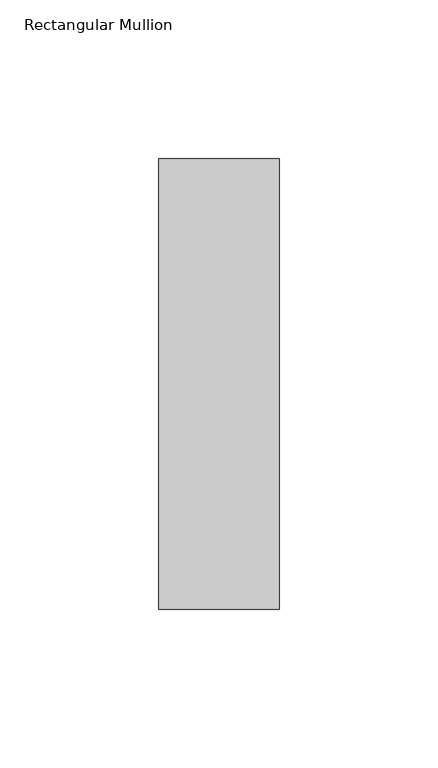
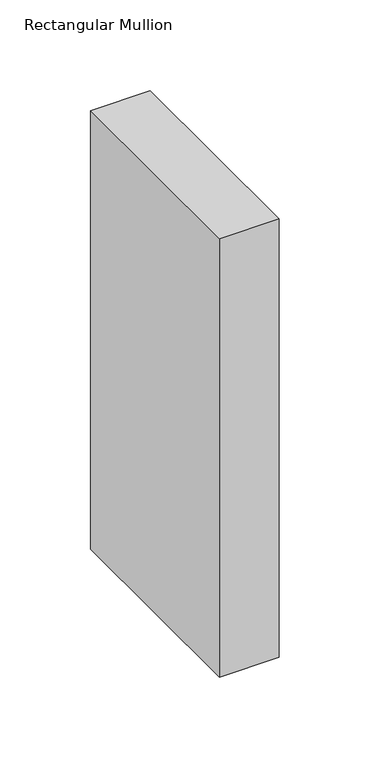
"""IFC4 building model written with IfcOpenShell, lengths in millimetres: member geometry, Rectangular Mullion : NLRS_21_CWM_hsb-regel 38x142_gen_rsf."""

import ifcopenshell
import ifcopenshell.guid

model = None  # the IFC model being written
_history = None  # IfcOwnerHistory: only IFC2X3 demands one
_inside = {}  # id of a spatial element -> (the spatial element, [elements in it])
_under = {}  # id of a project, library or spatial element -> (it, [spatial elements below it])
_declared = {}  # id of a project -> (the project, [libraries it declares])
_typed = {}  # id of a type object -> (the type object, [elements of that type])
_made_of = {}  # id of a material, layer set ... -> (it, [elements and type objects made of it])


def new_model(schema):
    """Start an empty IFC model of exactly this schema.

    Asked for "IFC4X3", IfcOpenShell would pick the latest addendum, in which some entities
    have other attributes; the version numbers below select the first issue.
    IFC2X3 requires an IfcOwnerHistory on every rooted entity: one is made here for all.
    """
    global model, _history
    if schema == "IFC4X3":
        model = ifcopenshell.file(schema_version=(4, 3, 0, 0))
    else:
        model = ifcopenshell.file(schema=schema)
    _inside.clear()
    _under.clear()
    _declared.clear()
    _typed.clear()
    _made_of.clear()
    _history = None
    if model.schema == "IFC2X3":
        org = make("IfcOrganization", Name="unknown")
        user = make(
            "IfcPersonAndOrganization",
            ThePerson=make("IfcPerson", FamilyName="unknown"),
            TheOrganization=org,
        )
        app = make(
            "IfcApplication",
            ApplicationDeveloper=org,
            Version="unknown",
            ApplicationFullName="unknown",
            ApplicationIdentifier="unknown",
        )
        _history = make(
            "IfcOwnerHistory",
            OwningUser=user,
            OwningApplication=app,
            ChangeAction="ADDED",
            CreationDate=0,
        )
    return model


def make(cls, **values):
    """One entity of the class cls with the attributes given. An attribute that is None is left unset."""
    return model.create_entity(
        cls, **{name: value for name, value in values.items() if value is not None}
    )


def rooted(cls, **values):
    """An entity with a GlobalId (a new one), such as an element, a storey or a relation."""
    return make(cls, GlobalId=ifcopenshell.guid.new(), OwnerHistory=_history, **values)


def si_unit(unit_type, name, prefix=None):
    """IfcSIUnit, for example si_unit("LENGTHUNIT", "METRE", prefix="MILLI")."""
    return make("IfcSIUnit", UnitType=unit_type, Prefix=prefix, Name=name)


def assignment(units):
    """IfcUnitAssignment: the units of a project."""
    return None if units is None else make("IfcUnitAssignment", Units=units)


def point(xyz):
    """IfcCartesianPoint."""
    return None if xyz is None else make("IfcCartesianPoint", Coordinates=xyz)


def direction(xyz):
    """IfcDirection."""
    return None if xyz is None else make("IfcDirection", DirectionRatios=xyz)


def frame(location, z_axis=None, x_axis=None):
    """IfcAxis2Placement3D, a coordinate frame: its origin and axes. An axis left out is left unset."""
    return make(
        "IfcAxis2Placement3D",
        Location=point(location),
        Axis=direction(z_axis),
        RefDirection=direction(x_axis),
    )


def origin():
    """The frame at (0, 0, 0) with its axes left unset."""
    return frame((0.0, 0.0, 0.0))


def place(relative_to, where):
    """IfcLocalPlacement: puts the frame where relative to a parent placement (None: the world)."""
    return make(
        "IfcLocalPlacement", PlacementRelTo=relative_to, RelativePlacement=where
    )


def context(
    kind, dimensions, precision=None, world=None, true_north=None, identifier=None
):
    """IfcGeometricRepresentationContext, for example the 3D "Model" context."""
    return make(
        "IfcGeometricRepresentationContext",
        ContextIdentifier=identifier,
        ContextType=kind,
        CoordinateSpaceDimension=dimensions,
        Precision=precision,
        WorldCoordinateSystem=world,
        TrueNorth=true_north,
    )


def project(units=None, contexts=None):
    """IfcProject with its units and contexts."""
    return rooted(
        "IfcProject",
        Name="project",
        RepresentationContexts=contexts,
        UnitsInContext=assignment(units),
    )


def spatial(cls, under=None, at=None, **own):
    """A site, building, storey or space (cls), placed at a placement, below another one or the project."""
    s = rooted(cls, ObjectPlacement=at, **own)
    if under is not None:
        _under.setdefault(under.id(), (under, []))[1].append(s)
    return s


def polyline(points):
    """IfcPolyline through the points."""
    return make("IfcPolyline", Points=[point(p) for p in points])


def outline(outer, holes=None, kind="AREA"):
    """IfcArbitraryClosedProfileDef: a profile drawn as a closed curve; with holes, ...WithVoids."""
    if holes is None:
        return make("IfcArbitraryClosedProfileDef", ProfileType=kind, OuterCurve=outer)
    return make(
        "IfcArbitraryProfileDefWithVoids",
        ProfileType=kind,
        OuterCurve=outer,
        InnerCurves=holes,
    )


def extrude(swept, where, along, depth):
    """IfcExtrudedAreaSolid: the profile swept, set in the frame where, extruded along a direction by depth."""
    return make(
        "IfcExtrudedAreaSolid",
        SweptArea=swept,
        Position=where,
        ExtrudedDirection=direction(along),
        Depth=depth,
    )


def shape(context_of_items, identifier, shape_type, items):
    """IfcShapeRepresentation: the items that make up one representation, for example the "Body"."""
    return make(
        "IfcShapeRepresentation",
        ContextOfItems=context_of_items,
        RepresentationIdentifier=identifier,
        RepresentationType=shape_type,
        Items=items,
    )


def source(mapping_origin, context_of_items, identifier, shape_type, items):
    """IfcRepresentationMap: a shape defined once, which mapped items show again and again."""
    return make(
        "IfcRepresentationMap",
        MappingOrigin=mapping_origin,
        MappedRepresentation=shape(context_of_items, identifier, shape_type, items),
    )


def transform(
    local_origin,
    x_axis=None,
    y_axis=None,
    z_axis=None,
    scale=None,
    scale2=None,
    scale3=None,
    uniform=True,
):
    """IfcCartesianTransformationOperator3D, or its non-uniform kind. x_axis, y_axis, z_axis: its Axis1, 2, 3."""
    if uniform:
        return make(
            "IfcCartesianTransformationOperator3D",
            Axis1=direction(x_axis),
            Axis2=direction(y_axis),
            LocalOrigin=point(local_origin),
            Scale=scale,
            Axis3=direction(z_axis),
        )
    return make(
        "IfcCartesianTransformationOperator3DnonUniform",
        Axis1=direction(x_axis),
        Axis2=direction(y_axis),
        LocalOrigin=point(local_origin),
        Scale=scale,
        Axis3=direction(z_axis),
        Scale2=scale2,
        Scale3=scale3,
    )


def mapped(mapping_source, mapping_target):
    """IfcMappedItem: shows the shape of a source again, moved by a transform."""
    return make(
        "IfcMappedItem", MappingSource=mapping_source, MappingTarget=mapping_target
    )


def made_of(thing, what):
    """Note that an element or type object is made of a material, layer set ...; save() writes the relation."""
    if what is not None:
        _made_of.setdefault(what.id(), (what, []))[1].append(thing)
    return thing


def element(
    cls,
    number,
    at=None,
    inside=None,
    cuts=None,
    type_object=None,
    material=None,
    context=None,
    identifier="Body",
    shape_type=None,
    held_by="IfcProductDefinitionShape",
    body=None,
    shapes=None,
    **own,
):
    """One element of the class cls, such as IfcWall. Its Tag is "e" and its number.

    at: its placement. inside: the storey or other place that contains it. cuts: it is an
    opening in that element (IfcRelVoidsElement). A single representation is given by context,
    identifier, shape_type and body (its items); several are given by shapes. held_by: the class
    of the entity that holds the representations. save() writes the other relations.
    """
    e = rooted(cls, Tag="e%d" % number, ObjectPlacement=at, **own)
    if body is not None:
        shapes = [shape(context, identifier, shape_type, body)]
    if shapes is not None:
        e.Representation = make(held_by, Representations=shapes)
    if inside is not None:
        _inside.setdefault(inside.id(), (inside, []))[1].append(e)
    if cuts is not None:
        rooted(
            "IfcRelVoidsElement", RelatingBuildingElement=cuts, RelatedOpeningElement=e
        )
    if type_object is not None:
        _typed.setdefault(type_object.id(), (type_object, []))[1].append(e)
    return made_of(e, material)


def aggregate(whole, parts):
    """IfcRelAggregates: a whole, such as a stair, and the parts it consists of."""
    return rooted("IfcRelAggregates", RelatingObject=whole, RelatedObjects=parts)


def save(model, path):
    """Write the relations noted so far, then the file.

    IfcRelAggregates (storeys below a building ...), IfcRelContainedInSpatialStructure (elements
    in a storey), IfcRelDefinesByType, IfcRelAssociatesMaterial and IfcRelDeclares: one each for
    every whole, place, type object, material and project.
    """
    for whole, parts in _under.values():
        aggregate(whole, parts)
    for where, things in _inside.values():
        rooted(
            "IfcRelContainedInSpatialStructure",
            RelatedElements=things,
            RelatingStructure=where,
        )
    for kind, things in _typed.values():
        rooted("IfcRelDefinesByType", RelatedObjects=things, RelatingType=kind)
    for what, things in _made_of.values():
        rooted("IfcRelAssociatesMaterial", RelatedObjects=things, RelatingMaterial=what)
    for by, libraries in _declared.values():
        rooted("IfcRelDeclares", RelatingContext=by, RelatedDefinitions=libraries)
    model.write(path)


def rectangular_mullion_4ed20356(model_context):
    return source(origin(), model_context, "Body", "SweptSolid", [
        extrude(outline(polyline([(0.0, -71.0), (-38.0, -71.0), (-38.0, 71.0), (0.0, 71.0), (0.0, -71.0)])), frame((0.0, 0.0, -295.0), z_axis=(0.0, 0.0, 1.0), x_axis=(1.0, 0.0, 0.0)), (0.0, 0.0, 1.0), 295.0),
    ])


if __name__ == "__main__":
    model = new_model("IFC4")
    model_context = context("Model", 3, world=origin())
    ifc_project = project(units=[si_unit("LENGTHUNIT", "METRE", prefix="MILLI")], contexts=[model_context])
    site = spatial("IfcSite", under=ifc_project)
    building = spatial("IfcBuilding", under=site)
    placement = place(None, origin())
    rectangular_mullion_shape = rectangular_mullion_4ed20356(model_context)
    element("IfcMember", 1, ObjectType="Rectangular Mullion : NLRS_21_CWM_hsb-regel 38x142_gen_rsf", at=placement, inside=building, context=model_context, shape_type="MappedRepresentation", body=[
        mapped(rectangular_mullion_shape, transform((0.0, 0.0, 0.0), x_axis=(1.0, 0.0, 0.0), y_axis=(0.0, 1.0, 0.0), z_axis=(0.0, 0.0, 1.0))),
    ])
    save(model, "model.ifc")

# Revit data of these elements
# Type "Rectangular Mullion : NLRS_21_CWM_hsb-regel 38x142_gen_rsf"
#   Export Type to IFC As = "IfcWall"
#   Type IfcGUID = "07M7mRoiH1CR8m_RSKIwpF"
#   Assembly Code = "21.10"
#   built-in parameter 1007322 = 0.465879 (stored number, unit not read)
#   built-in parameter 1007321 = 0.062336 (stored number, unit not read)
#   built-in parameter 1007320 = 0.062336 (stored number, unit not read)
# Element 1 (IfcMember, "Rectangular Mullion : NLRS_21_CWM_hsb-regel 38x142_gen_rsf")
#   Materials on its faces: "NLRS_i2_hout naaldhout vuren_gen_rsf"
# Materials
#   "NLRS_i2_hout naaldhout vuren_gen_rsf": class "I - Hout", colour RGB 234 199 147, transparency 0, Keynote = "i2", Manufacturer = "Revit Standards Foundation", URL = "www.revitstandards.org", Description = "hout vuren", Cost = 0
